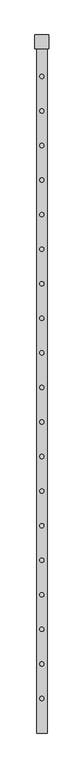
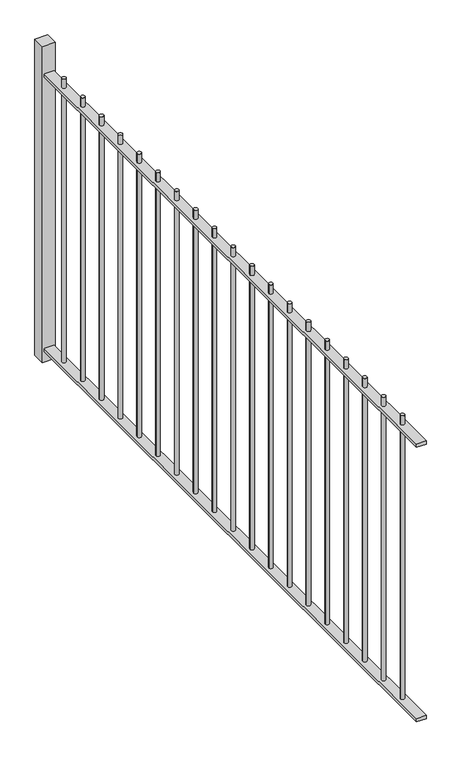
"""IFC4 building model written with IfcOpenShell, lengths in millimetres: railing geometry."""

from ifc_helpers import new_model, si_unit, point, frame, frame_2d, origin, place, context, project, spatial, polyline, circle_curve, trimmed, segment, composite_curve, outline, extrude, source, transform, mapped, element, save


def railing_b5f4cd0c(model_context):
    return source(origin(), model_context, "Body", "SweptSolid", [
        extrude(outline(polyline([(-6549.419961, -20891.1119119), (-6489.419961, -20891.1119119), (-6489.419961, -24891.1119119), (-6549.419961, -24891.1119119), (-6549.419961, -20891.1119119)])), frame((0.0, 0.0, -30.0), z_axis=(0.0, 0.0, 1.0), x_axis=(1.0, 0.0, 0.0)), (0.0, 0.0, 1.0), 20.0),
        extrude(outline(polyline([(-6549.419961, -20891.1119119), (-6489.419961, -20891.1119119), (-6489.419961, -24891.1119119), (-6549.419961, -24891.1119119), (-6549.419961, -20891.1119119)])), frame((0.0, 0.0, 1750.0), z_axis=(0.0, 0.0, 1.0), x_axis=(1.0, 0.0, 0.0)), (0.0, 0.0, 1.0), 20.0),
        extrude(outline(composite_curve([segment(trimmed(circle_curve(frame_2d((-6519.419961, -24691.1119119)), 12.5), [point((-6531.919961, -24691.1119119))], [point((-6506.919961, -24691.1119119))], False, "CARTESIAN"), True, "CONTINUOUS"), segment(trimmed(circle_curve(frame_2d((-6519.419961, -24691.1119119)), 12.5), [point((-6506.919961, -24691.1119119))], [point((-6531.919961, -24691.1119119))], False, "CARTESIAN"), True, "CONTINUOUS")], self_intersect=False)), frame((0.0, 0.0, -10.0), z_axis=(0.0, 0.0, 1.0), x_axis=(1.0, 0.0, 0.0)), (0.0, 0.0, 1.0), 1840.0),
        extrude(outline(composite_curve([segment(trimmed(circle_curve(frame_2d((-6519.419961, -24491.1119119)), 12.5), [point((-6531.919961, -24491.1119119))], [point((-6506.919961, -24491.1119119))], False, "CARTESIAN"), True, "CONTINUOUS"), segment(trimmed(circle_curve(frame_2d((-6519.419961, -24491.1119119)), 12.5), [point((-6506.919961, -24491.1119119))], [point((-6531.919961, -24491.1119119))], False, "CARTESIAN"), True, "CONTINUOUS")], self_intersect=False)), frame((0.0, 0.0, -10.0), z_axis=(0.0, 0.0, 1.0), x_axis=(1.0, 0.0, 0.0)), (0.0, 0.0, 1.0), 1840.0),
        extrude(outline(composite_curve([segment(trimmed(circle_curve(frame_2d((-6519.419961, -24291.1119119)), 12.5), [point((-6531.919961, -24291.1119119))], [point((-6506.919961, -24291.1119119))], False, "CARTESIAN"), True, "CONTINUOUS"), segment(trimmed(circle_curve(frame_2d((-6519.419961, -24291.1119119)), 12.5), [point((-6506.919961, -24291.1119119))], [point((-6531.919961, -24291.1119119))], False, "CARTESIAN"), True, "CONTINUOUS")], self_intersect=False)), frame((0.0, 0.0, -10.0), z_axis=(0.0, 0.0, 1.0), x_axis=(1.0, 0.0, 0.0)), (0.0, 0.0, 1.0), 1840.0),
        extrude(outline(composite_curve([segment(trimmed(circle_curve(frame_2d((-6519.419961, -24091.1119119)), 12.5), [point((-6531.919961, -24091.1119119))], [point((-6506.919961, -24091.1119119))], False, "CARTESIAN"), True, "CONTINUOUS"), segment(trimmed(circle_curve(frame_2d((-6519.419961, -24091.1119119)), 12.5), [point((-6506.919961, -24091.1119119))], [point((-6531.919961, -24091.1119119))], False, "CARTESIAN"), True, "CONTINUOUS")], self_intersect=False)), frame((0.0, 0.0, -10.0), z_axis=(0.0, 0.0, 1.0), x_axis=(1.0, 0.0, 0.0)), (0.0, 0.0, 1.0), 1840.0),
        extrude(outline(composite_curve([segment(trimmed(circle_curve(frame_2d((-6519.419961, -23891.1119119)), 12.5), [point((-6531.919961, -23891.1119119))], [point((-6506.919961, -23891.1119119))], False, "CARTESIAN"), True, "CONTINUOUS"), segment(trimmed(circle_curve(frame_2d((-6519.419961, -23891.1119119)), 12.5), [point((-6506.919961, -23891.1119119))], [point((-6531.919961, -23891.1119119))], False, "CARTESIAN"), True, "CONTINUOUS")], self_intersect=False)), frame((0.0, 0.0, -10.0), z_axis=(0.0, 0.0, 1.0), x_axis=(1.0, 0.0, 0.0)), (0.0, 0.0, 1.0), 1840.0),
        extrude(outline(composite_curve([segment(trimmed(circle_curve(frame_2d((-6519.419961, -23691.1119119)), 12.5), [point((-6531.919961, -23691.1119119))], [point((-6506.919961, -23691.1119119))], False, "CARTESIAN"), True, "CONTINUOUS"), segment(trimmed(circle_curve(frame_2d((-6519.419961, -23691.1119119)), 12.5), [point((-6506.919961, -23691.1119119))], [point((-6531.919961, -23691.1119119))], False, "CARTESIAN"), True, "CONTINUOUS")], self_intersect=False)), frame((0.0, 0.0, -10.0), z_axis=(0.0, 0.0, 1.0), x_axis=(1.0, 0.0, 0.0)), (0.0, 0.0, 1.0), 1840.0),
        extrude(outline(composite_curve([segment(trimmed(circle_curve(frame_2d((-6519.419961, -23491.1119119)), 12.5), [point((-6531.919961, -23491.1119119))], [point((-6506.919961, -23491.1119119))], False, "CARTESIAN"), True, "CONTINUOUS"), segment(trimmed(circle_curve(frame_2d((-6519.419961, -23491.1119119)), 12.5), [point((-6506.919961, -23491.1119119))], [point((-6531.919961, -23491.1119119))], False, "CARTESIAN"), True, "CONTINUOUS")], self_intersect=False)), frame((0.0, 0.0, -10.0), z_axis=(0.0, 0.0, 1.0), x_axis=(1.0, 0.0, 0.0)), (0.0, 0.0, 1.0), 1840.0),
        extrude(outline(composite_curve([segment(trimmed(circle_curve(frame_2d((-6519.419961, -23291.1119119)), 12.5), [point((-6531.919961, -23291.1119119))], [point((-6506.919961, -23291.1119119))], False, "CARTESIAN"), True, "CONTINUOUS"), segment(trimmed(circle_curve(frame_2d((-6519.419961, -23291.1119119)), 12.5), [point((-6506.919961, -23291.1119119))], [point((-6531.919961, -23291.1119119))], False, "CARTESIAN"), True, "CONTINUOUS")], self_intersect=False)), frame((0.0, 0.0, -10.0), z_axis=(0.0, 0.0, 1.0), x_axis=(1.0, 0.0, 0.0)), (0.0, 0.0, 1.0), 1840.0),
        extrude(outline(composite_curve([segment(trimmed(circle_curve(frame_2d((-6519.419961, -23091.1119119)), 12.5), [point((-6531.919961, -23091.1119119))], [point((-6506.919961, -23091.1119119))], False, "CARTESIAN"), True, "CONTINUOUS"), segment(trimmed(circle_curve(frame_2d((-6519.419961, -23091.1119119)), 12.5), [point((-6506.919961, -23091.1119119))], [point((-6531.919961, -23091.1119119))], False, "CARTESIAN"), True, "CONTINUOUS")], self_intersect=False)), frame((0.0, 0.0, -10.0), z_axis=(0.0, 0.0, 1.0), x_axis=(1.0, 0.0, 0.0)), (0.0, 0.0, 1.0), 1840.0),
        extrude(outline(composite_curve([segment(trimmed(circle_curve(frame_2d((-6519.419961, -22891.1119119)), 12.5), [point((-6531.919961, -22891.1119119))], [point((-6506.919961, -22891.1119119))], False, "CARTESIAN"), True, "CONTINUOUS"), segment(trimmed(circle_curve(frame_2d((-6519.419961, -22891.1119119)), 12.5), [point((-6506.919961, -22891.1119119))], [point((-6531.919961, -22891.1119119))], False, "CARTESIAN"), True, "CONTINUOUS")], self_intersect=False)), frame((0.0, 0.0, -10.0), z_axis=(0.0, 0.0, 1.0), x_axis=(1.0, 0.0, 0.0)), (0.0, 0.0, 1.0), 1840.0),
        extrude(outline(composite_curve([segment(trimmed(circle_curve(frame_2d((-6519.419961, -22691.1119119)), 12.5), [point((-6531.919961, -22691.1119119))], [point((-6506.919961, -22691.1119119))], False, "CARTESIAN"), True, "CONTINUOUS"), segment(trimmed(circle_curve(frame_2d((-6519.419961, -22691.1119119)), 12.5), [point((-6506.919961, -22691.1119119))], [point((-6531.919961, -22691.1119119))], False, "CARTESIAN"), True, "CONTINUOUS")], self_intersect=False)), frame((0.0, 0.0, -10.0), z_axis=(0.0, 0.0, 1.0), x_axis=(1.0, 0.0, 0.0)), (0.0, 0.0, 1.0), 1840.0),
        extrude(outline(composite_curve([segment(trimmed(circle_curve(frame_2d((-6519.419961, -22491.1119119)), 12.5), [point((-6531.919961, -22491.1119119))], [point((-6506.919961, -22491.1119119))], False, "CARTESIAN"), True, "CONTINUOUS"), segment(trimmed(circle_curve(frame_2d((-6519.419961, -22491.1119119)), 12.5), [point((-6506.919961, -22491.1119119))], [point((-6531.919961, -22491.1119119))], False, "CARTESIAN"), True, "CONTINUOUS")], self_intersect=False)), frame((0.0, 0.0, -10.0), z_axis=(0.0, 0.0, 1.0), x_axis=(1.0, 0.0, 0.0)), (0.0, 0.0, 1.0), 1840.0),
        extrude(outline(composite_curve([segment(trimmed(circle_curve(frame_2d((-6519.419961, -22291.1119119)), 12.5), [point((-6531.919961, -22291.1119119))], [point((-6506.919961, -22291.1119119))], False, "CARTESIAN"), True, "CONTINUOUS"), segment(trimmed(circle_curve(frame_2d((-6519.419961, -22291.1119119)), 12.5), [point((-6506.919961, -22291.1119119))], [point((-6531.919961, -22291.1119119))], False, "CARTESIAN"), True, "CONTINUOUS")], self_intersect=False)), frame((0.0, 0.0, -10.0), z_axis=(0.0, 0.0, 1.0), x_axis=(1.0, 0.0, 0.0)), (0.0, 0.0, 1.0), 1840.0),
        extrude(outline(composite_curve([segment(trimmed(circle_curve(frame_2d((-6519.419961, -22091.1119119)), 12.5), [point((-6531.919961, -22091.1119119))], [point((-6506.919961, -22091.1119119))], False, "CARTESIAN"), True, "CONTINUOUS"), segment(trimmed(circle_curve(frame_2d((-6519.419961, -22091.1119119)), 12.5), [point((-6506.919961, -22091.1119119))], [point((-6531.919961, -22091.1119119))], False, "CARTESIAN"), True, "CONTINUOUS")], self_intersect=False)), frame((0.0, 0.0, -10.0), z_axis=(0.0, 0.0, 1.0), x_axis=(1.0, 0.0, 0.0)), (0.0, 0.0, 1.0), 1840.0),
        extrude(outline(composite_curve([segment(trimmed(circle_curve(frame_2d((-6519.419961, -21891.1119119)), 12.5), [point((-6531.919961, -21891.1119119))], [point((-6506.919961, -21891.1119119))], False, "CARTESIAN"), True, "CONTINUOUS"), segment(trimmed(circle_curve(frame_2d((-6519.419961, -21891.1119119)), 12.5), [point((-6506.919961, -21891.1119119))], [point((-6531.919961, -21891.1119119))], False, "CARTESIAN"), True, "CONTINUOUS")], self_intersect=False)), frame((0.0, 0.0, -10.0), z_axis=(0.0, 0.0, 1.0), x_axis=(1.0, 0.0, 0.0)), (0.0, 0.0, 1.0), 1840.0),
        extrude(outline(composite_curve([segment(trimmed(circle_curve(frame_2d((-6519.419961, -21691.1119119)), 12.5), [point((-6531.919961, -21691.1119119))], [point((-6506.919961, -21691.1119119))], False, "CARTESIAN"), True, "CONTINUOUS"), segment(trimmed(circle_curve(frame_2d((-6519.419961, -21691.1119119)), 12.5), [point((-6506.919961, -21691.1119119))], [point((-6531.919961, -21691.1119119))], False, "CARTESIAN"), True, "CONTINUOUS")], self_intersect=False)), frame((0.0, 0.0, -10.0), z_axis=(0.0, 0.0, 1.0), x_axis=(1.0, 0.0, 0.0)), (0.0, 0.0, 1.0), 1840.0),
        extrude(outline(composite_curve([segment(trimmed(circle_curve(frame_2d((-6519.419961, -21491.1119119)), 12.5), [point((-6531.919961, -21491.1119119))], [point((-6506.919961, -21491.1119119))], False, "CARTESIAN"), True, "CONTINUOUS"), segment(trimmed(circle_curve(frame_2d((-6519.419961, -21491.1119119)), 12.5), [point((-6506.919961, -21491.1119119))], [point((-6531.919961, -21491.1119119))], False, "CARTESIAN"), True, "CONTINUOUS")], self_intersect=False)), frame((0.0, 0.0, -10.0), z_axis=(0.0, 0.0, 1.0), x_axis=(1.0, 0.0, 0.0)), (0.0, 0.0, 1.0), 1840.0),
        extrude(outline(composite_curve([segment(trimmed(circle_curve(frame_2d((-6519.419961, -21291.1119119)), 12.5), [point((-6531.919961, -21291.1119119))], [point((-6506.919961, -21291.1119119))], False, "CARTESIAN"), True, "CONTINUOUS"), segment(trimmed(circle_curve(frame_2d((-6519.419961, -21291.1119119)), 12.5), [point((-6506.919961, -21291.1119119))], [point((-6531.919961, -21291.1119119))], False, "CARTESIAN"), True, "CONTINUOUS")], self_intersect=False)), frame((0.0, 0.0, -10.0), z_axis=(0.0, 0.0, 1.0), x_axis=(1.0, 0.0, 0.0)), (0.0, 0.0, 1.0), 1840.0),
        extrude(outline(composite_curve([segment(trimmed(circle_curve(frame_2d((-6519.419961, -21091.1119119)), 12.5), [point((-6531.919961, -21091.1119119))], [point((-6506.919961, -21091.1119119))], False, "CARTESIAN"), True, "CONTINUOUS"), segment(trimmed(circle_curve(frame_2d((-6519.419961, -21091.1119119)), 12.5), [point((-6506.919961, -21091.1119119))], [point((-6531.919961, -21091.1119119))], False, "CARTESIAN"), True, "CONTINUOUS")], self_intersect=False)), frame((0.0, 0.0, -10.0), z_axis=(0.0, 0.0, 1.0), x_axis=(1.0, 0.0, 0.0)), (0.0, 0.0, 1.0), 1840.0),
        extrude(outline(polyline([(-6479.419961, -20851.1119119), (-6479.419961, -20931.1119119), (-6559.419961, -20931.1119119), (-6559.419961, -20851.1119119), (-6479.419961, -20851.1119119)])), frame((0.0, 0.0, -100.0), z_axis=(0.0, 0.0, 1.0), x_axis=(1.0, 0.0, 0.0)), (0.0, 0.0, 1.0), 2050.0),
    ])


if __name__ == "__main__":
    model = new_model("IFC4")
    model_context = context("Model", 3, world=origin())
    ifc_project = project(units=[si_unit("LENGTHUNIT", "METRE", prefix="MILLI")], contexts=[model_context])
    site = spatial("IfcSite", under=ifc_project)
    building = spatial("IfcBuilding", under=site)
    placement = place(None, origin())
    railing_shape = railing_b5f4cd0c(model_context)
    element("IfcRailing", 1, at=placement, inside=building, context=model_context, shape_type="MappedRepresentation", body=[
        mapped(railing_shape, transform((0.0, 0.0, 0.0), x_axis=(1.0, 0.0, 0.0), y_axis=(0.0, 1.0, 0.0), z_axis=(0.0, 0.0, 1.0))),
    ])
    save(model, "model.ifc")

# Revit data of these elements
# Element 1 (IfcRailing)
#   Materials on its faces: "NLRS_h2_staal_generiek zwart_gen_rsf", "NLRS_h2_staal_gen_rsf"
# Materials
#   "NLRS_h2_staal_generiek zwart_gen_rsf": class "Metal", colour RGB 189 187 185, transparency 0, Manufacturer = "RevitGG", URL = "www.revitgg.nl", Description = "Staal, generiek materiaal", Cost = 0
#   "NLRS_h2_staal_gen_rsf": class "H - Metaal", colour RGB 189 187 185, transparency 0, Keynote = "h2", Model = "generiek", Manufacturer = "Revit Standards Foundation", URL = "www.revitstandards.org", Description = "staal", Cost = 0
